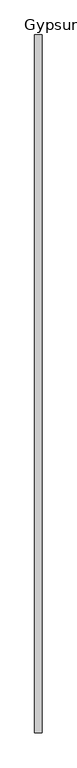
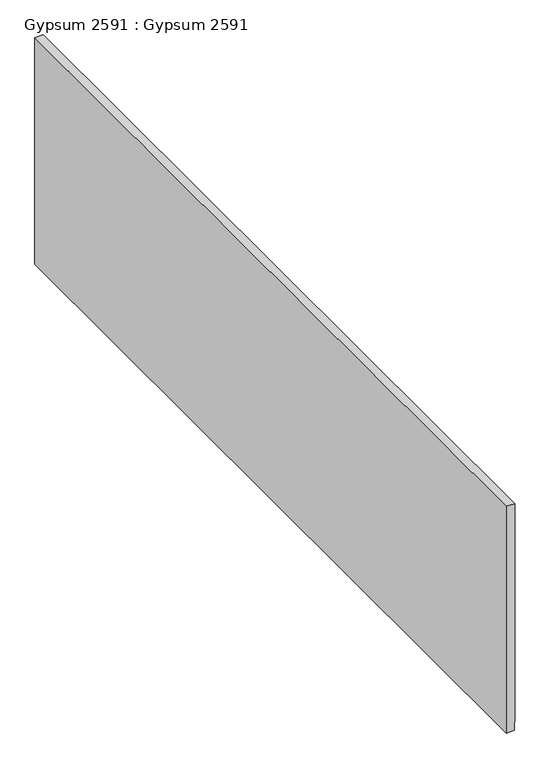
"""IFC4 building model written with IfcOpenShell, lengths in millimetres: proxy geometry, Gypsum 2591 : Gypsum 2591."""

from ifc_helpers import new_model, si_unit, frame, origin, place, context, project, spatial, polyline, outline, extrude, source, transform, mapped, element, save


def gypsum_2591_gypsum_2591_eb470674(model_context):
    return source(origin(), model_context, "Body", "SweptSolid", [
        extrude(outline(polyline([(39545.1675708, -640.491476), (39567.6883323, -640.491476), (39567.6883323, -639.211476), (40131.746, -639.211476), (40131.746, -660.156476), (39545.1675708, -660.156476), (39545.1675708, -640.491476)])), frame((0.0, -1052.8906574, 0.0), z_axis=(0.0, 1.0, 0.0), x_axis=(0.0, 0.0, 1.0)), (0.0, 0.0, 1.0), 2000.0),
    ])


if __name__ == "__main__":
    model = new_model("IFC4")
    model_context = context("Model", 3, world=origin())
    ifc_project = project(units=[si_unit("LENGTHUNIT", "METRE", prefix="MILLI")], contexts=[model_context])
    site = spatial("IfcSite", under=ifc_project)
    building = spatial("IfcBuilding", under=site)
    placement = place(None, origin())
    gypsum_2591_gypsum_2591_shape = gypsum_2591_gypsum_2591_eb470674(model_context)
    element("IfcBuildingElementProxy", 1, Name="Gypsum 2591 : Gypsum 2591", ObjectType="Gypsum 2591 : Gypsum 2591", at=placement, inside=building, context=model_context, shape_type="MappedRepresentation", body=[
        mapped(gypsum_2591_gypsum_2591_shape, transform((0.0, 0.0, 0.0), x_axis=(1.0, 0.0, 0.0), y_axis=(0.0, 1.0, 0.0), z_axis=(0.0, 0.0, 1.0))),
    ])
    save(model, "model.ifc")

# Revit data of these elements
# Type "Gypsum 2591 : Gypsum 2591"
#   NameOverride = "Gypsum"
# Element 1 (IfcBuildingElementProxy, "Gypsum 2591 : Gypsum 2591")
#   Materials on its faces: "5/8\" GYPSUM BOARD"
# Materials
#   "5/8\" GYPSUM BOARD": class "Unassigned", colour RGB 255 255 255, transparency 0, Cost = 0
